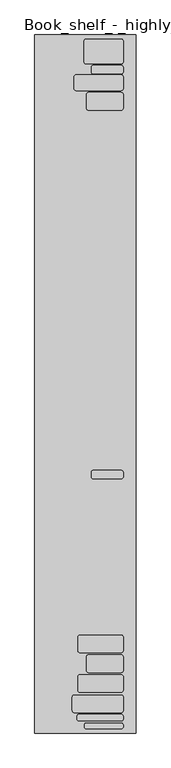
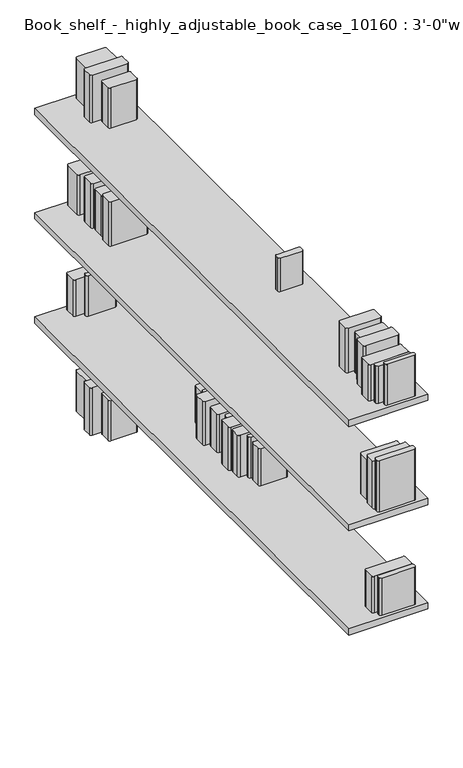
"""IFC4 building model written with IfcOpenShell, lengths in millimetres: furniture geometry."""

from ifc_helpers import new_model, si_unit, point, frame, frame_2d, origin, place, context, project, spatial, polyline, circle_curve, trimmed, segment, composite_curve, outline, extrude, source, transform, mapped, element, save


def furniture_7717bf60(model_context):
    return source(origin(), model_context, "Body", "SweptSolid", [
        extrude(outline(composite_curve([segment(polyline([(-148.9022418, 1904.6275375), (-148.9022418, 1945.1318477)]), True, "CONTINUOUS"), segment(trimmed(circle_curve(frame_2d((-142.5522418, 1945.1318477)), 6.35), [point((-148.9022418, 1945.1318477))], [point((-142.5522418, 1951.4818477))], False, "CARTESIAN"), True, "CONTINUOUS"), segment(polyline([(-142.5522418, 1951.4818477), (-44.45, 1951.4818477)]), True, "CONTINUOUS"), segment(trimmed(circle_curve(frame_2d((-44.45, 1945.1318477)), 6.35), [point((-44.45, 1951.4818477))], [point((-38.1, 1945.1318477))], False, "CARTESIAN"), True, "CONTINUOUS"), segment(polyline([(-38.1, 1945.1318477), (-38.1, 1904.6275375)]), True, "CONTINUOUS"), segment(trimmed(circle_curve(frame_2d((-44.45, 1904.6275375)), 6.35), [point((-38.1, 1904.6275375))], [point((-44.45, 1898.2775375))], False, "CARTESIAN"), True, "CONTINUOUS"), segment(polyline([(-44.45, 1898.2775375), (-142.5522418, 1898.2775375)]), True, "CONTINUOUS"), segment(trimmed(circle_curve(frame_2d((-142.5522418, 1904.6275375)), 6.35), [point((-142.5522418, 1898.2775375))], [point((-148.9022418, 1904.6275375))], False, "CARTESIAN"), True, "CONTINUOUS")], self_intersect=False)), frame((0.0, 0.0, 2254.0), z_axis=(0.0, 0.0, 1.0), x_axis=(1.0, 0.0, 0.0)), (0.0, 0.0, 1.0), 163.8466778),
        extrude(outline(composite_curve([segment(polyline([(-186.6960646, 1963.7563445), (-186.6960646, 1997.8877722)]), True, "CONTINUOUS"), segment(trimmed(circle_curve(frame_2d((-180.3460646, 1997.8877722)), 6.35), [point((-186.6960646, 1997.8877722))], [point((-180.3460646, 2004.2377722))], False, "CARTESIAN"), True, "CONTINUOUS"), segment(polyline([(-180.3460646, 2004.2377722), (-44.45, 2004.2377722)]), True, "CONTINUOUS"), segment(trimmed(circle_curve(frame_2d((-44.45, 1997.8877722)), 6.35), [point((-44.45, 2004.2377722))], [point((-38.1, 1997.8877722))], False, "CARTESIAN"), True, "CONTINUOUS"), segment(polyline([(-38.1, 1997.8877722), (-38.1, 1963.7563445)]), True, "CONTINUOUS"), segment(trimmed(circle_curve(frame_2d((-44.45, 1963.7563445)), 6.35), [point((-38.1, 1963.7563445))], [point((-44.45, 1957.4063445))], False, "CARTESIAN"), True, "CONTINUOUS"), segment(polyline([(-44.45, 1957.4063445), (-180.3460646, 1957.4063445)]), True, "CONTINUOUS"), segment(trimmed(circle_curve(frame_2d((-180.3460646, 1963.7563445)), 6.35), [point((-180.3460646, 1957.4063445))], [point((-186.6960646, 1963.7563445))], False, "CARTESIAN"), True, "CONTINUOUS")], self_intersect=False)), frame((0.0, 0.0, 2254.0), z_axis=(0.0, 0.0, 1.0), x_axis=(1.0, 0.0, 0.0)), (0.0, 0.0, 1.0), 193.2682698),
        extrude(outline(composite_curve([segment(polyline([(-156.1010652, 2043.8512848), (-156.1010652, 2105.55)]), True, "CONTINUOUS"), segment(trimmed(circle_curve(frame_2d((-149.7510652, 2105.55)), 6.35), [point((-156.1010652, 2105.55))], [point((-149.7510652, 2111.9))], False, "CARTESIAN"), True, "CONTINUOUS"), segment(polyline([(-149.7510652, 2111.9), (-44.45, 2111.9)]), True, "CONTINUOUS"), segment(trimmed(circle_curve(frame_2d((-44.45, 2105.55)), 6.35), [point((-44.45, 2111.9))], [point((-38.1, 2105.55))], False, "CARTESIAN"), True, "CONTINUOUS"), segment(polyline([(-38.1, 2105.55), (-38.1, 2043.8512848)]), True, "CONTINUOUS"), segment(trimmed(circle_curve(frame_2d((-44.45, 2043.8512848)), 6.35), [point((-38.1, 2043.8512848))], [point((-44.45, 2037.5012848))], False, "CARTESIAN"), True, "CONTINUOUS"), segment(polyline([(-44.45, 2037.5012848), (-149.7510652, 2037.5012848)]), True, "CONTINUOUS"), segment(trimmed(circle_curve(frame_2d((-149.7510652, 2043.8512848)), 6.35), [point((-149.7510652, 2037.5012848))], [point((-156.1010652, 2043.8512848))], False, "CARTESIAN"), True, "CONTINUOUS")], self_intersect=False)), frame((0.0, 0.0, 2254.0), z_axis=(0.0, 0.0, 1.0), x_axis=(1.0, 0.0, 0.0)), (0.0, 0.0, 1.0), 163.8466778),
        extrude(outline(composite_curve([segment(polyline([(-134.504595, 2013.7627722), (-134.504595, 2026.4627722)]), True, "CONTINUOUS"), segment(trimmed(circle_curve(frame_2d((-128.154595, 2026.4627722)), 6.35), [point((-134.504595, 2026.4627722))], [point((-128.154595, 2032.8127722))], False, "CARTESIAN"), True, "CONTINUOUS"), segment(polyline([(-128.154595, 2032.8127722), (-44.45, 2032.8127722)]), True, "CONTINUOUS"), segment(trimmed(circle_curve(frame_2d((-44.45, 2026.4627722)), 6.35), [point((-44.45, 2032.8127722))], [point((-38.1, 2026.4627722))], False, "CARTESIAN"), True, "CONTINUOUS"), segment(polyline([(-38.1, 2026.4627722), (-38.1, 2013.7627722)]), True, "CONTINUOUS"), segment(trimmed(circle_curve(frame_2d((-44.45, 2013.7627722)), 6.35), [point((-38.1, 2013.7627722))], [point((-44.45, 2007.4127722))], False, "CARTESIAN"), True, "CONTINUOUS"), segment(polyline([(-44.45, 2007.4127722), (-128.154595, 2007.4127722)]), True, "CONTINUOUS"), segment(trimmed(circle_curve(frame_2d((-128.154595, 2013.7627722)), 6.35), [point((-128.154595, 2007.4127722))], [point((-134.504595, 2013.7627722))], False, "CARTESIAN"), True, "CONTINUOUS")], self_intersect=False)), frame((0.0, 0.0, 2254.0), z_axis=(0.0, 0.0, 1.0), x_axis=(1.0, 0.0, 0.0)), (0.0, 0.0, 1.0), 135.8183694),
        extrude(outline(composite_curve([segment(polyline([(-174.9979766, 273.5343096), (-174.9979766, 313.4842776)]), True, "CONTINUOUS"), segment(trimmed(circle_curve(frame_2d((-168.6479766, 313.4842776)), 6.35), [point((-174.9979766, 313.4842776))], [point((-168.6479766, 319.8342776))], False, "CARTESIAN"), True, "CONTINUOUS"), segment(polyline([(-168.6479766, 319.8342776), (-44.45, 319.8342776)]), True, "CONTINUOUS"), segment(trimmed(circle_curve(frame_2d((-44.45, 313.4842776)), 6.35), [point((-44.45, 319.8342776))], [point((-38.1, 313.4842776))], False, "CARTESIAN"), True, "CONTINUOUS"), segment(polyline([(-38.1, 313.4842776), (-38.1, 273.5343096)]), True, "CONTINUOUS"), segment(trimmed(circle_curve(frame_2d((-44.45, 273.5343096)), 6.35), [point((-38.1, 273.5343096))], [point((-44.45, 267.1843096))], False, "CARTESIAN"), True, "CONTINUOUS"), segment(polyline([(-44.45, 267.1843096), (-168.6479766, 267.1843096)]), True, "CONTINUOUS"), segment(trimmed(circle_curve(frame_2d((-168.6479766, 273.5343096)), 6.35), [point((-168.6479766, 267.1843096))], [point((-174.9979766, 273.5343096))], False, "CARTESIAN"), True, "CONTINUOUS")], self_intersect=False)), frame((0.0, 0.0, 2254.0), z_axis=(0.0, 0.0, 1.0), x_axis=(1.0, 0.0, 0.0)), (0.0, 0.0, 1.0), 181.3914823),
        extrude(outline(composite_curve([segment(polyline([(-134.504595, 796.0843096), (-134.504595, 808.7843096)]), True, "CONTINUOUS"), segment(trimmed(circle_curve(frame_2d((-128.154595, 808.7843096)), 6.35), [point((-134.504595, 808.7843096))], [point((-128.154595, 815.1343096))], False, "CARTESIAN"), True, "CONTINUOUS"), segment(polyline([(-128.154595, 815.1343096), (-44.45, 815.1343096)]), True, "CONTINUOUS"), segment(trimmed(circle_curve(frame_2d((-44.45, 808.7843096)), 6.35), [point((-44.45, 815.1343096))], [point((-38.1, 808.7843096))], False, "CARTESIAN"), True, "CONTINUOUS"), segment(polyline([(-38.1, 808.7843096), (-38.1, 796.0843096)]), True, "CONTINUOUS"), segment(trimmed(circle_curve(frame_2d((-44.45, 796.0843096)), 6.35), [point((-38.1, 796.0843096))], [point((-44.45, 789.7343096))], False, "CARTESIAN"), True, "CONTINUOUS"), segment(polyline([(-44.45, 789.7343096), (-128.154595, 789.7343096)]), True, "CONTINUOUS"), segment(trimmed(circle_curve(frame_2d((-128.154595, 796.0843096)), 6.35), [point((-128.154595, 789.7343096))], [point((-134.504595, 796.0843096))], False, "CARTESIAN"), True, "CONTINUOUS")], self_intersect=False)), frame((0.0, 0.0, 2254.0), z_axis=(0.0, 0.0, 1.0), x_axis=(1.0, 0.0, 0.0)), (0.0, 0.0, 1.0), 135.8183694),
        extrude(outline(composite_curve([segment(polyline([(-174.9979766, 154.4873472), (-174.9979766, 194.4373151)]), True, "CONTINUOUS"), segment(trimmed(circle_curve(frame_2d((-168.6479766, 194.4373151)), 6.35), [point((-174.9979766, 194.4373151))], [point((-168.6479766, 200.7873151))], False, "CARTESIAN"), True, "CONTINUOUS"), segment(polyline([(-168.6479766, 200.7873151), (-44.45, 200.7873151)]), True, "CONTINUOUS"), segment(trimmed(circle_curve(frame_2d((-44.45, 194.4373151)), 6.35), [point((-44.45, 200.7873151))], [point((-38.1, 194.4373151))], False, "CARTESIAN"), True, "CONTINUOUS"), segment(polyline([(-38.1, 194.4373151), (-38.1, 154.4873472)]), True, "CONTINUOUS"), segment(trimmed(circle_curve(frame_2d((-44.45, 154.4873472)), 6.35), [point((-38.1, 154.4873472))], [point((-44.45, 148.1373472))], False, "CARTESIAN"), True, "CONTINUOUS"), segment(polyline([(-44.45, 148.1373472), (-168.6479766, 148.1373472)]), True, "CONTINUOUS"), segment(trimmed(circle_curve(frame_2d((-168.6479766, 154.4873472)), 6.35), [point((-168.6479766, 148.1373472))], [point((-174.9979766, 154.4873472))], False, "CARTESIAN"), True, "CONTINUOUS")], self_intersect=False)), frame((0.0, 0.0, 2254.0), z_axis=(0.0, 0.0, 1.0), x_axis=(1.0, 0.0, 0.0)), (0.0, 0.0, 1.0), 181.3914823),
        extrude(outline(composite_curve([segment(polyline([(-148.9022418, 213.6855624), (-148.9022418, 254.1898725)]), True, "CONTINUOUS"), segment(trimmed(circle_curve(frame_2d((-142.5522418, 254.1898725)), 6.35), [point((-148.9022418, 254.1898725))], [point((-142.5522418, 260.5398725))], False, "CARTESIAN"), True, "CONTINUOUS"), segment(polyline([(-142.5522418, 260.5398725), (-44.45, 260.5398725)]), True, "CONTINUOUS"), segment(trimmed(circle_curve(frame_2d((-44.45, 254.1898725)), 6.35), [point((-44.45, 260.5398725))], [point((-38.1, 254.1898725))], False, "CARTESIAN"), True, "CONTINUOUS"), segment(polyline([(-38.1, 254.1898725), (-38.1, 213.6855624)]), True, "CONTINUOUS"), segment(trimmed(circle_curve(frame_2d((-44.45, 213.6855624)), 6.35), [point((-38.1, 213.6855624))], [point((-44.45, 207.3355624))], False, "CARTESIAN"), True, "CONTINUOUS"), segment(polyline([(-44.45, 207.3355624), (-142.5522418, 207.3355624)]), True, "CONTINUOUS"), segment(trimmed(circle_curve(frame_2d((-142.5522418, 213.6855624)), 6.35), [point((-142.5522418, 207.3355624))], [point((-148.9022418, 213.6855624))], False, "CARTESIAN"), True, "CONTINUOUS")], self_intersect=False)), frame((0.0, 0.0, 2254.0), z_axis=(0.0, 0.0, 1.0), x_axis=(1.0, 0.0, 0.0)), (0.0, 0.0, 1.0), 163.8466778),
        extrude(outline(composite_curve([segment(polyline([(-155.6511388, 44.45), (-155.6511388, 48.7119243)]), True, "CONTINUOUS"), segment(trimmed(circle_curve(frame_2d((-149.3011388, 48.7119243)), 6.35), [point((-155.6511388, 48.7119243))], [point((-149.3011388, 55.0619243))], False, "CARTESIAN"), True, "CONTINUOUS"), segment(polyline([(-149.3011388, 55.0619243), (-44.45, 55.0619243)]), True, "CONTINUOUS"), segment(trimmed(circle_curve(frame_2d((-44.45, 48.7119243)), 6.35), [point((-44.45, 55.0619243))], [point((-38.1, 48.7119243))], False, "CARTESIAN"), True, "CONTINUOUS"), segment(polyline([(-38.1, 48.7119243), (-38.1, 44.45)]), True, "CONTINUOUS"), segment(trimmed(circle_curve(frame_2d((-44.45, 44.45)), 6.35), [point((-38.1, 44.45))], [point((-44.45, 38.1))], False, "CARTESIAN"), True, "CONTINUOUS"), segment(polyline([(-44.45, 38.1), (-149.3011388, 38.1)]), True, "CONTINUOUS"), segment(trimmed(circle_curve(frame_2d((-149.3011388, 44.45)), 6.35), [point((-149.3011388, 38.1))], [point((-155.6511388, 44.45))], False, "CARTESIAN"), True, "CONTINUOUS")], self_intersect=False)), frame((0.0, 0.0, 2254.0), z_axis=(0.0, 0.0, 1.0), x_axis=(1.0, 0.0, 0.0)), (0.0, 0.0, 1.0), 166.2690481),
        extrude(outline(composite_curve([segment(polyline([(-191.8289872, 93.2744988), (-191.8289872, 133.2244668)]), True, "CONTINUOUS"), segment(trimmed(circle_curve(frame_2d((-185.4789872, 133.2244668)), 6.35), [point((-191.8289872, 133.2244668))], [point((-185.4789872, 139.5744668))], False, "CARTESIAN"), True, "CONTINUOUS"), segment(polyline([(-185.4789872, 139.5744668), (-44.45, 139.5744668)]), True, "CONTINUOUS"), segment(trimmed(circle_curve(frame_2d((-44.45, 133.2244668)), 6.35), [point((-44.45, 139.5744668))], [point((-38.1, 133.2244668))], False, "CARTESIAN"), True, "CONTINUOUS"), segment(polyline([(-38.1, 133.2244668), (-38.1, 93.2744988)]), True, "CONTINUOUS"), segment(trimmed(circle_curve(frame_2d((-44.45, 93.2744988)), 6.35), [point((-38.1, 93.2744988))], [point((-44.45, 86.9244988))], False, "CARTESIAN"), True, "CONTINUOUS"), segment(polyline([(-44.45, 86.9244988), (-185.4789872, 86.9244988)]), True, "CONTINUOUS"), segment(trimmed(circle_curve(frame_2d((-185.4789872, 93.2744988)), 6.35), [point((-185.4789872, 86.9244988))], [point((-191.8289872, 93.2744988))], False, "CARTESIAN"), True, "CONTINUOUS")], self_intersect=False)), frame((0.0, 0.0, 2254.0), z_axis=(0.0, 0.0, 1.0), x_axis=(1.0, 0.0, 0.0)), (0.0, 0.0, 1.0), 148.7566688),
        extrude(outline(composite_curve([segment(polyline([(-177.3825869, 67.874514), (-177.3825869, 75.2798723)]), True, "CONTINUOUS"), segment(trimmed(circle_curve(frame_2d((-171.0325869, 75.2798723)), 6.35), [point((-177.3825869, 75.2798723))], [point((-171.0325869, 81.6298723))], False, "CARTESIAN"), True, "CONTINUOUS"), segment(polyline([(-171.0325869, 81.6298723), (-44.45, 81.6298723)]), True, "CONTINUOUS"), segment(trimmed(circle_curve(frame_2d((-44.45, 75.2798723)), 6.35), [point((-44.45, 81.6298723))], [point((-38.1, 75.2798723))], False, "CARTESIAN"), True, "CONTINUOUS"), segment(polyline([(-38.1, 75.2798723), (-38.1, 67.874514)]), True, "CONTINUOUS"), segment(trimmed(circle_curve(frame_2d((-44.45, 67.874514)), 6.35), [point((-38.1, 67.874514))], [point((-44.45, 61.524514))], False, "CARTESIAN"), True, "CONTINUOUS"), segment(polyline([(-44.45, 61.524514), (-171.0325869, 61.524514)]), True, "CONTINUOUS"), segment(trimmed(circle_curve(frame_2d((-171.0325869, 67.874514)), 6.35), [point((-171.0325869, 61.524514))], [point((-177.3825869, 67.874514))], False, "CARTESIAN"), True, "CONTINUOUS")], self_intersect=False)), frame((0.0, 0.0, 2254.0), z_axis=(0.0, 0.0, 1.0), x_axis=(1.0, 0.0, 0.0)), (0.0, 0.0, 1.0), 151.8618711),
        extrude(outline(polyline([(0.0, 2124.6), (0.0, 25.4), (-304.8, 25.4), (-304.8, 2124.6), (0.0, 2124.6)])), frame((0.0, 0.0, 2228.6), z_axis=(0.0, 0.0, 1.0), x_axis=(1.0, 0.0, 0.0)), (0.0, 0.0, 1.0), 25.4),
        extrude(outline(composite_curve([segment(polyline([(-181.0020996, 119.7389676), (-181.0020996, 160.2432777)]), True, "CONTINUOUS"), segment(trimmed(circle_curve(frame_2d((-174.6520996, 160.2432777)), 6.35), [point((-181.0020996, 160.2432777))], [point((-174.6520996, 166.5932777))], False, "CARTESIAN"), True, "CONTINUOUS"), segment(polyline([(-174.6520996, 166.5932777), (-44.45, 166.5932777)]), True, "CONTINUOUS"), segment(trimmed(circle_curve(frame_2d((-44.45, 160.2432777)), 6.35), [point((-44.45, 166.5932777))], [point((-38.1, 160.2432777))], False, "CARTESIAN"), True, "CONTINUOUS"), segment(polyline([(-38.1, 160.2432777), (-38.1, 119.7389676)]), True, "CONTINUOUS"), segment(trimmed(circle_curve(frame_2d((-44.45, 119.7389676)), 6.35), [point((-38.1, 119.7389676))], [point((-44.45, 113.3889676))], False, "CARTESIAN"), True, "CONTINUOUS"), segment(polyline([(-44.45, 113.3889676), (-174.6520996, 113.3889676)]), True, "CONTINUOUS"), segment(trimmed(circle_curve(frame_2d((-174.6520996, 119.7389676)), 6.35), [point((-174.6520996, 113.3889676))], [point((-181.0020996, 119.7389676))], False, "CARTESIAN"), True, "CONTINUOUS")], self_intersect=False)), frame((0.0, 0.0, 1828.6), z_axis=(0.0, 0.0, 1.0), x_axis=(1.0, 0.0, 0.0)), (0.0, 0.0, 1.0), 163.8466778),
        extrude(outline(composite_curve([segment(polyline([(-187.30107, 1955.1650696), (-187.30107, 1995.1150375)]), True, "CONTINUOUS"), segment(trimmed(circle_curve(frame_2d((-180.95107, 1995.1150375)), 6.35), [point((-187.30107, 1995.1150375))], [point((-180.95107, 2001.4650375))], False, "CARTESIAN"), True, "CONTINUOUS"), segment(polyline([(-180.95107, 2001.4650375), (-44.45, 2001.4650375)]), True, "CONTINUOUS"), segment(trimmed(circle_curve(frame_2d((-44.45, 1995.1150375)), 6.35), [point((-44.45, 2001.4650375))], [point((-38.1, 1995.1150375))], False, "CARTESIAN"), True, "CONTINUOUS"), segment(polyline([(-38.1, 1995.1150375), (-38.1, 1955.1650696)]), True, "CONTINUOUS"), segment(trimmed(circle_curve(frame_2d((-44.45, 1955.1650696)), 6.35), [point((-38.1, 1955.1650696))], [point((-44.45, 1948.8150696))], False, "CARTESIAN"), True, "CONTINUOUS"), segment(polyline([(-44.45, 1948.8150696), (-180.95107, 1948.8150696)]), True, "CONTINUOUS"), segment(trimmed(circle_curve(frame_2d((-180.95107, 1955.1650696)), 6.35), [point((-180.95107, 1948.8150696))], [point((-187.30107, 1955.1650696))], False, "CARTESIAN"), True, "CONTINUOUS")], self_intersect=False)), frame((0.0, 0.0, 1828.6), z_axis=(0.0, 0.0, 1.0), x_axis=(1.0, 0.0, 0.0)), (0.0, 0.0, 1.0), 181.3914823),
        extrude(outline(composite_curve([segment(polyline([(-186.4012171, 44.45), (-186.4012171, 53.326397)]), True, "CONTINUOUS"), segment(trimmed(circle_curve(frame_2d((-180.0512171, 53.326397)), 6.35), [point((-186.4012171, 53.326397))], [point((-180.0512171, 59.676397))], False, "CARTESIAN"), True, "CONTINUOUS"), segment(polyline([(-180.0512171, 59.676397), (-44.45, 59.676397)]), True, "CONTINUOUS"), segment(trimmed(circle_curve(frame_2d((-44.45, 53.326397)), 6.35), [point((-44.45, 59.676397))], [point((-38.1, 53.326397))], False, "CARTESIAN"), True, "CONTINUOUS"), segment(polyline([(-38.1, 53.326397), (-38.1, 44.45)]), True, "CONTINUOUS"), segment(trimmed(circle_curve(frame_2d((-44.45, 44.45)), 6.35), [point((-38.1, 44.45))], [point((-44.45, 38.1))], False, "CARTESIAN"), True, "CONTINUOUS"), segment(polyline([(-44.45, 38.1), (-180.0512171, 38.1)]), True, "CONTINUOUS"), segment(trimmed(circle_curve(frame_2d((-180.0512171, 44.45)), 6.35), [point((-180.0512171, 38.1))], [point((-186.4012171, 44.45))], False, "CARTESIAN"), True, "CONTINUOUS")], self_intersect=False)), frame((0.0, 0.0, 1828.6), z_axis=(0.0, 0.0, 1.0), x_axis=(1.0, 0.0, 0.0)), (0.0, 0.0, 1.0), 209.55),
        extrude(outline(composite_curve([segment(polyline([(-189.1007759, 68.366525), (-189.1007759, 102.4979527)]), True, "CONTINUOUS"), segment(trimmed(circle_curve(frame_2d((-182.7507759, 102.4979527)), 6.35), [point((-189.1007759, 102.4979527))], [point((-182.7507759, 108.8479527))], False, "CARTESIAN"), True, "CONTINUOUS"), segment(polyline([(-182.7507759, 108.8479527), (-44.45, 108.8479527)]), True, "CONTINUOUS"), segment(trimmed(circle_curve(frame_2d((-44.45, 102.4979527)), 6.35), [point((-44.45, 108.8479527))], [point((-38.1, 102.4979527))], False, "CARTESIAN"), True, "CONTINUOUS"), segment(polyline([(-38.1, 102.4979527), (-38.1, 68.366525)]), True, "CONTINUOUS"), segment(trimmed(circle_curve(frame_2d((-44.45, 68.366525)), 6.35), [point((-38.1, 68.366525))], [point((-44.45, 62.016525))], False, "CARTESIAN"), True, "CONTINUOUS"), segment(polyline([(-44.45, 62.016525), (-182.7507759, 62.016525)]), True, "CONTINUOUS"), segment(trimmed(circle_curve(frame_2d((-182.7507759, 68.366525)), 6.35), [point((-182.7507759, 62.016525))], [point((-189.1007759, 68.366525))], False, "CARTESIAN"), True, "CONTINUOUS")], self_intersect=False)), frame((0.0, 0.0, 1828.6), z_axis=(0.0, 0.0, 1.0), x_axis=(1.0, 0.0, 0.0)), (0.0, 0.0, 1.0), 193.2682698),
        extrude(outline(composite_curve([segment(polyline([(-172.0035703, 2011.3075348), (-172.0035703, 2024.0075348)]), True, "CONTINUOUS"), segment(trimmed(circle_curve(frame_2d((-165.6535703, 2024.0075348)), 6.35), [point((-172.0035703, 2024.0075348))], [point((-165.6535703, 2030.3575348))], False, "CARTESIAN"), True, "CONTINUOUS"), segment(polyline([(-165.6535703, 2030.3575348), (-44.45, 2030.3575348)]), True, "CONTINUOUS"), segment(trimmed(circle_curve(frame_2d((-44.45, 2024.0075348)), 6.35), [point((-44.45, 2030.3575348))], [point((-38.1, 2024.0075348))], False, "CARTESIAN"), True, "CONTINUOUS"), segment(polyline([(-38.1, 2024.0075348), (-38.1, 2011.3075348)]), True, "CONTINUOUS"), segment(trimmed(circle_curve(frame_2d((-44.45, 2011.3075348)), 6.35), [point((-38.1, 2011.3075348))], [point((-44.45, 2004.9575348))], False, "CARTESIAN"), True, "CONTINUOUS"), segment(polyline([(-44.45, 2004.9575348), (-165.6535703, 2004.9575348)]), True, "CONTINUOUS"), segment(trimmed(circle_curve(frame_2d((-165.6535703, 2011.3075348)), 6.35), [point((-165.6535703, 2004.9575348))], [point((-172.0035703, 2011.3075348))], False, "CARTESIAN"), True, "CONTINUOUS")], self_intersect=False)), frame((0.0, 0.0, 1828.6), z_axis=(0.0, 0.0, 1.0), x_axis=(1.0, 0.0, 0.0)), (0.0, 0.0, 1.0), 135.8183694),
        extrude(outline(composite_curve([segment(polyline([(-188.4046355, 2043.8512848), (-188.4046355, 2105.55)]), True, "CONTINUOUS"), segment(trimmed(circle_curve(frame_2d((-182.0546355, 2105.55)), 6.35), [point((-188.4046355, 2105.55))], [point((-182.0546355, 2111.9))], False, "CARTESIAN"), True, "CONTINUOUS"), segment(polyline([(-182.0546355, 2111.9), (-44.45, 2111.9)]), True, "CONTINUOUS"), segment(trimmed(circle_curve(frame_2d((-44.45, 2105.55)), 6.35), [point((-44.45, 2111.9))], [point((-38.1, 2105.55))], False, "CARTESIAN"), True, "CONTINUOUS"), segment(polyline([(-38.1, 2105.55), (-38.1, 2043.8512848)]), True, "CONTINUOUS"), segment(trimmed(circle_curve(frame_2d((-44.45, 2043.8512848)), 6.35), [point((-38.1, 2043.8512848))], [point((-44.45, 2037.5012848))], False, "CARTESIAN"), True, "CONTINUOUS"), segment(polyline([(-44.45, 2037.5012848), (-182.0546355, 2037.5012848)]), True, "CONTINUOUS"), segment(trimmed(circle_curve(frame_2d((-182.0546355, 2043.8512848)), 6.35), [point((-182.0546355, 2037.5012848))], [point((-188.4046355, 2043.8512848))], False, "CARTESIAN"), True, "CONTINUOUS")], self_intersect=False)), frame((0.0, 0.0, 1828.6), z_axis=(0.0, 0.0, 1.0), x_axis=(1.0, 0.0, 0.0)), (0.0, 0.0, 1.0), 163.8466778),
        extrude(outline(composite_curve([segment(polyline([(-187.30107, 1834.5150696), (-187.30107, 1874.4650375)]), True, "CONTINUOUS"), segment(trimmed(circle_curve(frame_2d((-180.95107, 1874.4650375)), 6.35), [point((-187.30107, 1874.4650375))], [point((-180.95107, 1880.8150375))], False, "CARTESIAN"), True, "CONTINUOUS"), segment(polyline([(-180.95107, 1880.8150375), (-44.45, 1880.8150375)]), True, "CONTINUOUS"), segment(trimmed(circle_curve(frame_2d((-44.45, 1874.4650375)), 6.35), [point((-44.45, 1880.8150375))], [point((-38.1, 1874.4650375))], False, "CARTESIAN"), True, "CONTINUOUS"), segment(polyline([(-38.1, 1874.4650375), (-38.1, 1834.5150696)]), True, "CONTINUOUS"), segment(trimmed(circle_curve(frame_2d((-44.45, 1834.5150696)), 6.35), [point((-38.1, 1834.5150696))], [point((-44.45, 1828.1650696))], False, "CARTESIAN"), True, "CONTINUOUS"), segment(polyline([(-44.45, 1828.1650696), (-180.95107, 1828.1650696)]), True, "CONTINUOUS"), segment(trimmed(circle_curve(frame_2d((-180.95107, 1834.5150696)), 6.35), [point((-180.95107, 1828.1650696))], [point((-187.30107, 1834.5150696))], False, "CARTESIAN"), True, "CONTINUOUS")], self_intersect=False)), frame((0.0, 0.0, 1828.6), z_axis=(0.0, 0.0, 1.0), x_axis=(1.0, 0.0, 0.0)), (0.0, 0.0, 1.0), 181.3914823),
        extrude(outline(composite_curve([segment(polyline([(-181.0020996, 1895.4125122), (-181.0020996, 1935.9168223)]), True, "CONTINUOUS"), segment(trimmed(circle_curve(frame_2d((-174.6520996, 1935.9168223)), 6.35), [point((-181.0020996, 1935.9168223))], [point((-174.6520996, 1942.2668223))], False, "CARTESIAN"), True, "CONTINUOUS"), segment(polyline([(-174.6520996, 1942.2668223), (-44.45, 1942.2668223)]), True, "CONTINUOUS"), segment(trimmed(circle_curve(frame_2d((-44.45, 1935.9168223)), 6.35), [point((-44.45, 1942.2668223))], [point((-38.1, 1935.9168223))], False, "CARTESIAN"), True, "CONTINUOUS"), segment(polyline([(-38.1, 1935.9168223), (-38.1, 1895.4125122)]), True, "CONTINUOUS"), segment(trimmed(circle_curve(frame_2d((-44.45, 1895.4125122)), 6.35), [point((-38.1, 1895.4125122))], [point((-44.45, 1889.0625122))], False, "CARTESIAN"), True, "CONTINUOUS"), segment(polyline([(-44.45, 1889.0625122), (-174.6520996, 1889.0625122)]), True, "CONTINUOUS"), segment(trimmed(circle_curve(frame_2d((-174.6520996, 1895.4125122)), 6.35), [point((-174.6520996, 1889.0625122))], [point((-181.0020996, 1895.4125122))], False, "CARTESIAN"), True, "CONTINUOUS")], self_intersect=False)), frame((0.0, 0.0, 1828.6), z_axis=(0.0, 0.0, 1.0), x_axis=(1.0, 0.0, 0.0)), (0.0, 0.0, 1.0), 163.8466778),
        extrude(outline(polyline([(0.0, 2124.6), (0.0, 25.4), (-304.8, 25.4), (-304.8, 2124.6), (0.0, 2124.6)])), frame((0.0, 0.0, 1803.2), z_axis=(0.0, 0.0, 1.0), x_axis=(1.0, 0.0, 0.0)), (0.0, 0.0, 1.0), 25.4),
        extrude(outline(composite_curve([segment(polyline([(-149.8020947, 1282.3412422), (-149.8020947, 1317.9947053)]), True, "CONTINUOUS"), segment(trimmed(circle_curve(frame_2d((-143.4520947, 1317.9947053)), 6.35), [point((-149.8020947, 1317.9947053))], [point((-143.4520947, 1324.3447053))], False, "CARTESIAN"), True, "CONTINUOUS"), segment(polyline([(-143.4520947, 1324.3447053), (-44.45, 1324.3447053)]), True, "CONTINUOUS"), segment(trimmed(circle_curve(frame_2d((-44.45, 1317.9947053)), 6.35), [point((-44.45, 1324.3447053))], [point((-38.1, 1317.9947053))], False, "CARTESIAN"), True, "CONTINUOUS"), segment(polyline([(-38.1, 1317.9947053), (-38.1, 1282.3412422)]), True, "CONTINUOUS"), segment(trimmed(circle_curve(frame_2d((-44.45, 1282.3412422)), 6.35), [point((-38.1, 1282.3412422))], [point((-44.45, 1275.9912422))], False, "CARTESIAN"), True, "CONTINUOUS"), segment(polyline([(-44.45, 1275.9912422), (-143.4520947, 1275.9912422)]), True, "CONTINUOUS"), segment(trimmed(circle_curve(frame_2d((-143.4520947, 1282.3412422)), 6.35), [point((-143.4520947, 1275.9912422))], [point((-149.8020947, 1282.3412422))], False, "CARTESIAN"), True, "CONTINUOUS")], self_intersect=False)), frame((0.0, 0.0, 1403.2), z_axis=(0.0, 0.0, 1.0), x_axis=(1.0, 0.0, 0.0)), (0.0, 0.0, 1.0), 151.8506516),
        extrude(outline(composite_curve([segment(polyline([(-155.6511388, 1258.4604527), (-155.6511388, 1262.7223771)]), True, "CONTINUOUS"), segment(trimmed(circle_curve(frame_2d((-149.3011388, 1262.7223771)), 6.35), [point((-155.6511388, 1262.7223771))], [point((-149.3011388, 1269.0723771))], False, "CARTESIAN"), True, "CONTINUOUS"), segment(polyline([(-149.3011388, 1269.0723771), (-44.45, 1269.0723771)]), True, "CONTINUOUS"), segment(trimmed(circle_curve(frame_2d((-44.45, 1262.7223771)), 6.35), [point((-44.45, 1269.0723771))], [point((-38.1, 1262.7223771))], False, "CARTESIAN"), True, "CONTINUOUS"), segment(polyline([(-38.1, 1262.7223771), (-38.1, 1258.4604527)]), True, "CONTINUOUS"), segment(trimmed(circle_curve(frame_2d((-44.45, 1258.4604527)), 6.35), [point((-38.1, 1258.4604527))], [point((-44.45, 1252.1104527))], False, "CARTESIAN"), True, "CONTINUOUS"), segment(polyline([(-44.45, 1252.1104527), (-149.3011388, 1252.1104527)]), True, "CONTINUOUS"), segment(trimmed(circle_curve(frame_2d((-149.3011388, 1258.4604527)), 6.35), [point((-149.3011388, 1252.1104527))], [point((-155.6511388, 1258.4604527))], False, "CARTESIAN"), True, "CONTINUOUS")], self_intersect=False)), frame((0.0, 0.0, 1403.2), z_axis=(0.0, 0.0, 1.0), x_axis=(1.0, 0.0, 0.0)), (0.0, 0.0, 1.0), 166.2690481),
        extrude(outline(composite_curve([segment(polyline([(-191.8289872, 1198.562532), (-191.8289872, 1238.5125)]), True, "CONTINUOUS"), segment(trimmed(circle_curve(frame_2d((-185.4789872, 1238.5125)), 6.35), [point((-191.8289872, 1238.5125))], [point((-185.4789872, 1244.8625))], False, "CARTESIAN"), True, "CONTINUOUS"), segment(polyline([(-185.4789872, 1244.8625), (-44.45, 1244.8625)]), True, "CONTINUOUS"), segment(trimmed(circle_curve(frame_2d((-44.45, 1238.5125)), 6.35), [point((-44.45, 1244.8625))], [point((-38.1, 1238.5125))], False, "CARTESIAN"), True, "CONTINUOUS"), segment(polyline([(-38.1, 1238.5125), (-38.1, 1198.562532)]), True, "CONTINUOUS"), segment(trimmed(circle_curve(frame_2d((-44.45, 1198.562532)), 6.35), [point((-38.1, 1198.562532))], [point((-44.45, 1192.212532))], False, "CARTESIAN"), True, "CONTINUOUS"), segment(polyline([(-44.45, 1192.212532), (-185.4789872, 1192.212532)]), True, "CONTINUOUS"), segment(trimmed(circle_curve(frame_2d((-185.4789872, 1198.562532)), 6.35), [point((-185.4789872, 1192.212532))], [point((-191.8289872, 1198.562532))], False, "CARTESIAN"), True, "CONTINUOUS")], self_intersect=False)), frame((0.0, 0.0, 1402.9310239), z_axis=(0.0, 0.0, 1.0), x_axis=(1.0, 0.0, 0.0)), (0.0, 0.0, 1.0), 177.2506516),
        extrude(outline(composite_curve([segment(polyline([(-149.8020947, 900.375), (-149.8020947, 936.0284631)]), True, "CONTINUOUS"), segment(trimmed(circle_curve(frame_2d((-143.4520947, 936.0284631)), 6.35), [point((-149.8020947, 936.0284631))], [point((-143.4520947, 942.3784631))], False, "CARTESIAN"), True, "CONTINUOUS"), segment(polyline([(-143.4520947, 942.3784631), (-44.45, 942.3784631)]), True, "CONTINUOUS"), segment(trimmed(circle_curve(frame_2d((-44.45, 936.0284631)), 6.35), [point((-44.45, 942.3784631))], [point((-38.1, 936.0284631))], False, "CARTESIAN"), True, "CONTINUOUS"), segment(polyline([(-38.1, 936.0284631), (-38.1, 900.375)]), True, "CONTINUOUS"), segment(trimmed(circle_curve(frame_2d((-44.45, 900.375)), 6.35), [point((-38.1, 900.375))], [point((-44.45, 894.025))], False, "CARTESIAN"), True, "CONTINUOUS"), segment(polyline([(-44.45, 894.025), (-143.4520947, 894.025)]), True, "CONTINUOUS"), segment(trimmed(circle_curve(frame_2d((-143.4520947, 900.375)), 6.35), [point((-143.4520947, 894.025))], [point((-149.8020947, 900.375))], False, "CARTESIAN"), True, "CONTINUOUS")], self_intersect=False)), frame((0.0, 0.0, 1402.9310239), z_axis=(0.0, 0.0, 1.0), x_axis=(1.0, 0.0, 0.0)), (0.0, 0.0, 1.0), 151.8506516),
        extrude(outline(composite_curve([segment(polyline([(-155.6511388, 956.8354527), (-155.6511388, 961.0973771)]), True, "CONTINUOUS"), segment(trimmed(circle_curve(frame_2d((-149.3011388, 961.0973771)), 6.35), [point((-155.6511388, 961.0973771))], [point((-149.3011388, 967.4473771))], False, "CARTESIAN"), True, "CONTINUOUS"), segment(polyline([(-149.3011388, 967.4473771), (-44.45, 967.4473771)]), True, "CONTINUOUS"), segment(trimmed(circle_curve(frame_2d((-44.45, 961.0973771)), 6.35), [point((-44.45, 967.4473771))], [point((-38.1, 961.0973771))], False, "CARTESIAN"), True, "CONTINUOUS"), segment(polyline([(-38.1, 961.0973771), (-38.1, 956.8354527)]), True, "CONTINUOUS"), segment(trimmed(circle_curve(frame_2d((-44.45, 956.8354527)), 6.35), [point((-38.1, 956.8354527))], [point((-44.45, 950.4854527))], False, "CARTESIAN"), True, "CONTINUOUS"), segment(polyline([(-44.45, 950.4854527), (-149.3011388, 950.4854527)]), True, "CONTINUOUS"), segment(trimmed(circle_curve(frame_2d((-149.3011388, 956.8354527)), 6.35), [point((-149.3011388, 950.4854527))], [point((-155.6511388, 956.8354527))], False, "CARTESIAN"), True, "CONTINUOUS")], self_intersect=False)), frame((0.0, 0.0, 1403.2), z_axis=(0.0, 0.0, 1.0), x_axis=(1.0, 0.0, 0.0)), (0.0, 0.0, 1.0), 166.2690481),
        extrude(outline(composite_curve([segment(polyline([(-191.8289872, 2065.600032), (-191.8289872, 2105.55)]), True, "CONTINUOUS"), segment(trimmed(circle_curve(frame_2d((-185.4789872, 2105.55)), 6.35), [point((-191.8289872, 2105.55))], [point((-185.4789872, 2111.9))], False, "CARTESIAN"), True, "CONTINUOUS"), segment(polyline([(-185.4789872, 2111.9), (-44.45, 2111.9)]), True, "CONTINUOUS"), segment(trimmed(circle_curve(frame_2d((-44.45, 2105.55)), 6.35), [point((-44.45, 2111.9))], [point((-38.1, 2105.55))], False, "CARTESIAN"), True, "CONTINUOUS"), segment(polyline([(-38.1, 2105.55), (-38.1, 2065.600032)]), True, "CONTINUOUS"), segment(trimmed(circle_curve(frame_2d((-44.45, 2065.600032)), 6.35), [point((-38.1, 2065.600032))], [point((-44.45, 2059.250032))], False, "CARTESIAN"), True, "CONTINUOUS"), segment(polyline([(-44.45, 2059.250032), (-185.4789872, 2059.250032)]), True, "CONTINUOUS"), segment(trimmed(circle_curve(frame_2d((-185.4789872, 2065.600032)), 6.35), [point((-185.4789872, 2059.250032))], [point((-191.8289872, 2065.600032))], False, "CARTESIAN"), True, "CONTINUOUS")], self_intersect=False)), frame((0.0, 0.0, 1403.2), z_axis=(0.0, 0.0, 1.0), x_axis=(1.0, 0.0, 0.0)), (0.0, 0.0, 1.0), 148.7566688),
        extrude(outline(composite_curve([segment(polyline([(-155.6511388, 2044.962532), (-155.6511388, 2049.2244564)]), True, "CONTINUOUS"), segment(trimmed(circle_curve(frame_2d((-149.3011388, 2049.2244564)), 6.35), [point((-155.6511388, 2049.2244564))], [point((-149.3011388, 2055.5744564))], False, "CARTESIAN"), True, "CONTINUOUS"), segment(polyline([(-149.3011388, 2055.5744564), (-44.45, 2055.5744564)]), True, "CONTINUOUS"), segment(trimmed(circle_curve(frame_2d((-44.45, 2049.2244564)), 6.35), [point((-44.45, 2055.5744564))], [point((-38.1, 2049.2244564))], False, "CARTESIAN"), True, "CONTINUOUS"), segment(polyline([(-38.1, 2049.2244564), (-38.1, 2044.962532)]), True, "CONTINUOUS"), segment(trimmed(circle_curve(frame_2d((-44.45, 2044.962532)), 6.35), [point((-38.1, 2044.962532))], [point((-44.45, 2038.612532))], False, "CARTESIAN"), True, "CONTINUOUS"), segment(polyline([(-44.45, 2038.612532), (-149.3011388, 2038.612532)]), True, "CONTINUOUS"), segment(trimmed(circle_curve(frame_2d((-149.3011388, 2044.962532)), 6.35), [point((-149.3011388, 2038.612532))], [point((-155.6511388, 2044.962532))], False, "CARTESIAN"), True, "CONTINUOUS")], self_intersect=False)), frame((0.0, 0.0, 1403.2), z_axis=(0.0, 0.0, 1.0), x_axis=(1.0, 0.0, 0.0)), (0.0, 0.0, 1.0), 166.2690481),
        extrude(outline(composite_curve([segment(polyline([(-191.8289872, 69.8499848), (-191.8289872, 109.7999528)]), True, "CONTINUOUS"), segment(trimmed(circle_curve(frame_2d((-185.4789872, 109.7999528)), 6.35), [point((-191.8289872, 109.7999528))], [point((-185.4789872, 116.1499528))], False, "CARTESIAN"), True, "CONTINUOUS"), segment(polyline([(-185.4789872, 116.1499528), (-44.45, 116.1499528)]), True, "CONTINUOUS"), segment(trimmed(circle_curve(frame_2d((-44.45, 109.7999528)), 6.35), [point((-44.45, 116.1499528))], [point((-38.1, 109.7999528))], False, "CARTESIAN"), True, "CONTINUOUS"), segment(polyline([(-38.1, 109.7999528), (-38.1, 69.8499848)]), True, "CONTINUOUS"), segment(trimmed(circle_curve(frame_2d((-44.45, 69.8499848)), 6.35), [point((-38.1, 69.8499848))], [point((-44.45, 63.4999848))], False, "CARTESIAN"), True, "CONTINUOUS"), segment(polyline([(-44.45, 63.4999848), (-185.4789872, 63.4999848)]), True, "CONTINUOUS"), segment(trimmed(circle_curve(frame_2d((-185.4789872, 69.8499848)), 6.35), [point((-185.4789872, 63.4999848))], [point((-191.8289872, 69.8499848))], False, "CARTESIAN"), True, "CONTINUOUS")], self_intersect=False)), frame((0.0, 0.0, 1403.2), z_axis=(0.0, 0.0, 1.0), x_axis=(1.0, 0.0, 0.0)), (0.0, 0.0, 1.0), 148.7566688),
        extrude(outline(composite_curve([segment(polyline([(-177.3825869, 44.45), (-177.3825869, 51.8553582)]), True, "CONTINUOUS"), segment(trimmed(circle_curve(frame_2d((-171.0325869, 51.8553582)), 6.35), [point((-177.3825869, 51.8553582))], [point((-171.0325869, 58.2053582))], False, "CARTESIAN"), True, "CONTINUOUS"), segment(polyline([(-171.0325869, 58.2053582), (-44.45, 58.2053582)]), True, "CONTINUOUS"), segment(trimmed(circle_curve(frame_2d((-44.45, 51.8553582)), 6.35), [point((-44.45, 58.2053582))], [point((-38.1, 51.8553582))], False, "CARTESIAN"), True, "CONTINUOUS"), segment(polyline([(-38.1, 51.8553582), (-38.1, 44.45)]), True, "CONTINUOUS"), segment(trimmed(circle_curve(frame_2d((-44.45, 44.45)), 6.35), [point((-38.1, 44.45))], [point((-44.45, 38.1))], False, "CARTESIAN"), True, "CONTINUOUS"), segment(polyline([(-44.45, 38.1), (-171.0325869, 38.1)]), True, "CONTINUOUS"), segment(trimmed(circle_curve(frame_2d((-171.0325869, 44.45)), 6.35), [point((-171.0325869, 38.1))], [point((-177.3825869, 44.45))], False, "CARTESIAN"), True, "CONTINUOUS")], self_intersect=False)), frame((0.0, 0.0, 1403.2), z_axis=(0.0, 0.0, 1.0), x_axis=(1.0, 0.0, 0.0)), (0.0, 0.0, 1.0), 151.8618711),
        extrude(outline(composite_curve([segment(polyline([(-183.9965059, 979.75), (-183.9965059, 1011.5)]), True, "CONTINUOUS"), segment(trimmed(circle_curve(frame_2d((-177.6465059, 1011.5)), 6.35), [point((-183.9965059, 1011.5))], [point((-177.6465059, 1017.85))], False, "CARTESIAN"), True, "CONTINUOUS"), segment(polyline([(-177.6465059, 1017.85), (-44.45, 1017.85)]), True, "CONTINUOUS"), segment(trimmed(circle_curve(frame_2d((-44.45, 1011.5)), 6.35), [point((-44.45, 1017.85))], [point((-38.1, 1011.5))], False, "CARTESIAN"), True, "CONTINUOUS"), segment(polyline([(-38.1, 1011.5), (-38.1, 979.75)]), True, "CONTINUOUS"), segment(trimmed(circle_curve(frame_2d((-44.45, 979.75)), 6.35), [point((-38.1, 979.75))], [point((-44.45, 973.4))], False, "CARTESIAN"), True, "CONTINUOUS"), segment(polyline([(-44.45, 973.4), (-177.6465059, 973.4)]), True, "CONTINUOUS"), segment(trimmed(circle_curve(frame_2d((-177.6465059, 979.75)), 6.35), [point((-177.6465059, 973.4))], [point((-183.9965059, 979.75))], False, "CARTESIAN"), True, "CONTINUOUS")], self_intersect=False)), frame((0.0, 0.0, 1402.9310239), z_axis=(0.0, 0.0, 1.0), x_axis=(1.0, 0.0, 0.0)), (0.0, 0.0, 1.0), 170.2851068),
        extrude(outline(composite_curve([segment(polyline([(-149.8020947, 1084.525), (-149.8020947, 1120.1784631)]), True, "CONTINUOUS"), segment(trimmed(circle_curve(frame_2d((-143.4520947, 1120.1784631)), 6.35), [point((-149.8020947, 1120.1784631))], [point((-143.4520947, 1126.5284631))], False, "CARTESIAN"), True, "CONTINUOUS"), segment(polyline([(-143.4520947, 1126.5284631), (-44.45, 1126.5284631)]), True, "CONTINUOUS"), segment(trimmed(circle_curve(frame_2d((-44.45, 1120.1784631)), 6.35), [point((-44.45, 1126.5284631))], [point((-38.1, 1120.1784631))], False, "CARTESIAN"), True, "CONTINUOUS"), segment(polyline([(-38.1, 1120.1784631), (-38.1, 1084.525)]), True, "CONTINUOUS"), segment(trimmed(circle_curve(frame_2d((-44.45, 1084.525)), 6.35), [point((-38.1, 1084.525))], [point((-44.45, 1078.175))], False, "CARTESIAN"), True, "CONTINUOUS"), segment(polyline([(-44.45, 1078.175), (-143.4520947, 1078.175)]), True, "CONTINUOUS"), segment(trimmed(circle_curve(frame_2d((-143.4520947, 1084.525)), 6.35), [point((-143.4520947, 1078.175))], [point((-149.8020947, 1084.525))], False, "CARTESIAN"), True, "CONTINUOUS")], self_intersect=False)), frame((0.0, 0.0, 1402.9310239), z_axis=(0.0, 0.0, 1.0), x_axis=(1.0, 0.0, 0.0)), (0.0, 0.0, 1.0), 151.8506516),
        extrude(outline(composite_curve([segment(polyline([(-172.6452674, 1138.237532), (-172.6452674, 1178.1875)]), True, "CONTINUOUS"), segment(trimmed(circle_curve(frame_2d((-166.2952674, 1178.1875)), 6.35), [point((-172.6452674, 1178.1875))], [point((-166.2952674, 1184.5375))], False, "CARTESIAN"), True, "CONTINUOUS"), segment(polyline([(-166.2952674, 1184.5375), (-44.45, 1184.5375)]), True, "CONTINUOUS"), segment(trimmed(circle_curve(frame_2d((-44.45, 1178.1875)), 6.35), [point((-44.45, 1184.5375))], [point((-38.1, 1178.1875))], False, "CARTESIAN"), True, "CONTINUOUS"), segment(polyline([(-38.1, 1178.1875), (-38.1, 1138.237532)]), True, "CONTINUOUS"), segment(trimmed(circle_curve(frame_2d((-44.45, 1138.237532)), 6.35), [point((-38.1, 1138.237532))], [point((-44.45, 1131.887532))], False, "CARTESIAN"), True, "CONTINUOUS"), segment(polyline([(-44.45, 1131.887532), (-166.2952674, 1131.887532)]), True, "CONTINUOUS"), segment(trimmed(circle_curve(frame_2d((-166.2952674, 1138.237532)), 6.35), [point((-166.2952674, 1131.887532))], [point((-172.6452674, 1138.237532))], False, "CARTESIAN"), True, "CONTINUOUS")], self_intersect=False)), frame((0.0, 0.0, 1402.9310239), z_axis=(0.0, 0.0, 1.0), x_axis=(1.0, 0.0, 0.0)), (0.0, 0.0, 1.0), 157.0434797),
        extrude(outline(composite_curve([segment(polyline([(-191.8289872, 1028.700032), (-191.8289872, 1068.65)]), True, "CONTINUOUS"), segment(trimmed(circle_curve(frame_2d((-185.4789872, 1068.65)), 6.35), [point((-191.8289872, 1068.65))], [point((-185.4789872, 1075.0))], False, "CARTESIAN"), True, "CONTINUOUS"), segment(polyline([(-185.4789872, 1075.0), (-44.45, 1075.0)]), True, "CONTINUOUS"), segment(trimmed(circle_curve(frame_2d((-44.45, 1068.65)), 6.35), [point((-44.45, 1075.0))], [point((-38.1, 1068.65))], False, "CARTESIAN"), True, "CONTINUOUS"), segment(polyline([(-38.1, 1068.65), (-38.1, 1028.700032)]), True, "CONTINUOUS"), segment(trimmed(circle_curve(frame_2d((-44.45, 1028.700032)), 6.35), [point((-38.1, 1028.700032))], [point((-44.45, 1022.350032))], False, "CARTESIAN"), True, "CONTINUOUS"), segment(polyline([(-44.45, 1022.350032), (-185.4789872, 1022.350032)]), True, "CONTINUOUS"), segment(trimmed(circle_curve(frame_2d((-185.4789872, 1028.700032)), 6.35), [point((-185.4789872, 1022.350032))], [point((-191.8289872, 1028.700032))], False, "CARTESIAN"), True, "CONTINUOUS")], self_intersect=False)), frame((0.0, 0.0, 1402.9310239), z_axis=(0.0, 0.0, 1.0), x_axis=(1.0, 0.0, 0.0)), (0.0, 0.0, 1.0), 177.2506516),
        extrude(outline(polyline([(0.0, 2124.6), (0.0, 25.4), (-304.8, 25.4), (-304.8, 2124.6), (0.0, 2124.6)])), frame((0.0, 0.0, 1377.8), z_axis=(0.0, 0.0, 1.0), x_axis=(1.0, 0.0, 0.0)), (0.0, 0.0, 1.0), 25.4),
        extrude(outline(composite_curve([segment(polyline([(-148.9022418, 1904.6275375), (-148.9022418, 1945.1318477)]), True, "CONTINUOUS"), segment(trimmed(circle_curve(frame_2d((-142.5522418, 1945.1318477)), 6.35), [point((-148.9022418, 1945.1318477))], [point((-142.5522418, 1951.4818477))], False, "CARTESIAN"), True, "CONTINUOUS"), segment(polyline([(-142.5522418, 1951.4818477), (-44.45, 1951.4818477)]), True, "CONTINUOUS"), segment(trimmed(circle_curve(frame_2d((-44.45, 1945.1318477)), 6.35), [point((-44.45, 1951.4818477))], [point((-38.1, 1945.1318477))], False, "CARTESIAN"), True, "CONTINUOUS"), segment(polyline([(-38.1, 1945.1318477), (-38.1, 1904.6275375)]), True, "CONTINUOUS"), segment(trimmed(circle_curve(frame_2d((-44.45, 1904.6275375)), 6.35), [point((-38.1, 1904.6275375))], [point((-44.45, 1898.2775375))], False, "CARTESIAN"), True, "CONTINUOUS"), segment(polyline([(-44.45, 1898.2775375), (-142.5522418, 1898.2775375)]), True, "CONTINUOUS"), segment(trimmed(circle_curve(frame_2d((-142.5522418, 1904.6275375)), 6.35), [point((-142.5522418, 1898.2775375))], [point((-148.9022418, 1904.6275375))], False, "CARTESIAN"), True, "CONTINUOUS")], self_intersect=False)), frame((0.0, 0.0, 977.8), z_axis=(0.0, 0.0, 1.0), x_axis=(1.0, 0.0, 0.0)), (0.0, 0.0, 1.0), 163.8466778),
        extrude(outline(composite_curve([segment(polyline([(-186.6960646, 1963.7563445), (-186.6960646, 1997.8877722)]), True, "CONTINUOUS"), segment(trimmed(circle_curve(frame_2d((-180.3460646, 1997.8877722)), 6.35), [point((-186.6960646, 1997.8877722))], [point((-180.3460646, 2004.2377722))], False, "CARTESIAN"), True, "CONTINUOUS"), segment(polyline([(-180.3460646, 2004.2377722), (-44.45, 2004.2377722)]), True, "CONTINUOUS"), segment(trimmed(circle_curve(frame_2d((-44.45, 1997.8877722)), 6.35), [point((-44.45, 2004.2377722))], [point((-38.1, 1997.8877722))], False, "CARTESIAN"), True, "CONTINUOUS"), segment(polyline([(-38.1, 1997.8877722), (-38.1, 1963.7563445)]), True, "CONTINUOUS"), segment(trimmed(circle_curve(frame_2d((-44.45, 1963.7563445)), 6.35), [point((-38.1, 1963.7563445))], [point((-44.45, 1957.4063445))], False, "CARTESIAN"), True, "CONTINUOUS"), segment(polyline([(-44.45, 1957.4063445), (-180.3460646, 1957.4063445)]), True, "CONTINUOUS"), segment(trimmed(circle_curve(frame_2d((-180.3460646, 1963.7563445)), 6.35), [point((-180.3460646, 1957.4063445))], [point((-186.6960646, 1963.7563445))], False, "CARTESIAN"), True, "CONTINUOUS")], self_intersect=False)), frame((0.0, 0.0, 977.8), z_axis=(0.0, 0.0, 1.0), x_axis=(1.0, 0.0, 0.0)), (0.0, 0.0, 1.0), 193.2682698),
        extrude(outline(composite_curve([segment(polyline([(-156.1010652, 2043.8512848), (-156.1010652, 2105.55)]), True, "CONTINUOUS"), segment(trimmed(circle_curve(frame_2d((-149.7510652, 2105.55)), 6.35), [point((-156.1010652, 2105.55))], [point((-149.7510652, 2111.9))], False, "CARTESIAN"), True, "CONTINUOUS"), segment(polyline([(-149.7510652, 2111.9), (-44.45, 2111.9)]), True, "CONTINUOUS"), segment(trimmed(circle_curve(frame_2d((-44.45, 2105.55)), 6.35), [point((-44.45, 2111.9))], [point((-38.1, 2105.55))], False, "CARTESIAN"), True, "CONTINUOUS"), segment(polyline([(-38.1, 2105.55), (-38.1, 2043.8512848)]), True, "CONTINUOUS"), segment(trimmed(circle_curve(frame_2d((-44.45, 2043.8512848)), 6.35), [point((-38.1, 2043.8512848))], [point((-44.45, 2037.5012848))], False, "CARTESIAN"), True, "CONTINUOUS"), segment(polyline([(-44.45, 2037.5012848), (-149.7510652, 2037.5012848)]), True, "CONTINUOUS"), segment(trimmed(circle_curve(frame_2d((-149.7510652, 2043.8512848)), 6.35), [point((-149.7510652, 2037.5012848))], [point((-156.1010652, 2043.8512848))], False, "CARTESIAN"), True, "CONTINUOUS")], self_intersect=False)), frame((0.0, 0.0, 977.8), z_axis=(0.0, 0.0, 1.0), x_axis=(1.0, 0.0, 0.0)), (0.0, 0.0, 1.0), 163.8466778),
        extrude(outline(composite_curve([segment(polyline([(-134.504595, 2013.7627722), (-134.504595, 2026.4627722)]), True, "CONTINUOUS"), segment(trimmed(circle_curve(frame_2d((-128.154595, 2026.4627722)), 6.35), [point((-134.504595, 2026.4627722))], [point((-128.154595, 2032.8127722))], False, "CARTESIAN"), True, "CONTINUOUS"), segment(polyline([(-128.154595, 2032.8127722), (-44.45, 2032.8127722)]), True, "CONTINUOUS"), segment(trimmed(circle_curve(frame_2d((-44.45, 2026.4627722)), 6.35), [point((-44.45, 2032.8127722))], [point((-38.1, 2026.4627722))], False, "CARTESIAN"), True, "CONTINUOUS"), segment(polyline([(-38.1, 2026.4627722), (-38.1, 2013.7627722)]), True, "CONTINUOUS"), segment(trimmed(circle_curve(frame_2d((-44.45, 2013.7627722)), 6.35), [point((-38.1, 2013.7627722))], [point((-44.45, 2007.4127722))], False, "CARTESIAN"), True, "CONTINUOUS"), segment(polyline([(-44.45, 2007.4127722), (-128.154595, 2007.4127722)]), True, "CONTINUOUS"), segment(trimmed(circle_curve(frame_2d((-128.154595, 2013.7627722)), 6.35), [point((-128.154595, 2007.4127722))], [point((-134.504595, 2013.7627722))], False, "CARTESIAN"), True, "CONTINUOUS")], self_intersect=False)), frame((0.0, 0.0, 977.8), z_axis=(0.0, 0.0, 1.0), x_axis=(1.0, 0.0, 0.0)), (0.0, 0.0, 1.0), 135.8183694),
    ])


if __name__ == "__main__":
    model = new_model("IFC4")
    model_context = context("Model", 3, world=origin())
    ifc_project = project(units=[si_unit("LENGTHUNIT", "METRE", prefix="MILLI")], contexts=[model_context])
    site = spatial("IfcSite", under=ifc_project)
    building = spatial("IfcBuilding", under=site)
    placement = place(None, origin())
    furniture_shape = furniture_7717bf60(model_context)
    element("IfcFurniture", 1, ObjectType="Book_shelf_-_highly_adjustable_book_case_10160 : 3'-0\"w 6'-0\"h", at=placement, inside=building, context=model_context, shape_type="MappedRepresentation", body=[
        mapped(furniture_shape, transform((0.0, 0.0, 0.0), x_axis=(1.0, 0.0, 0.0), y_axis=(0.0, 1.0, 0.0), z_axis=(0.0, 0.0, 1.0))),
    ])
    save(model, "model.ifc")

# Revit data of these elements
# Type "Book_shelf_-_highly_adjustable_book_case_10160 : 3'-0\"w 6'-0\"h"
#   total height = 2.8 m
#   toe kick height = 0.1016 m
#   shelf width = 2.0992 m
#   shelf depth = 0.3048 m
#   shelf 6 bottom = 2.1016 m
#   shelf 5 height = 0.4 m
#   shelf 5 bottom = 1.6762 m
#   shelf 4 height = 0.4 m
#   shelf 4 bottom = 1.2508 m
#   shelf 3 height = 0.4 m
#   shelf 2 height = 0.4 m
#   shelf 1 height = 0.4 m
#   bookcase width = 2.15 m
#   shelf 3 bottom = 0.8254 m
#   shelf 6 = yes
#   shelf 5 = yes
#   shelf 4 = yes
#   shelf 3 = yes
#   shelf 2 books = yes
#   shelf 2 = yes
#   books = yes
#   bookcase back = yes
#   Book5 = book blue
#   Book4 = book red
#   Book3 = book green
#   Book2 = book red
#   Book1 = book light blue
#   Book Shelf = book white
#   Default Elevation = 0
# Element 1 (IfcFurniture, "Book_shelf_-_highly_adjustable_book_case_10160 : 3'-0\"w 6'-0\"h")
#   Materials on its faces: "book red", "book blue", "book green", "book light blue", "book white"
# Materials
#   "book blue": class "Paint", colour RGB 13 13 83, transparency 0
#   "book red": class "Paint", colour RGB 229 30 30, transparency 0
#   "book green": class "Paint", colour RGB 81 104 43, transparency 0
#   "book light blue": class "Paint", colour RGB 81 140 196, transparency 0
#   "book white": class "Paint", colour RGB 211 193 153, transparency 0
